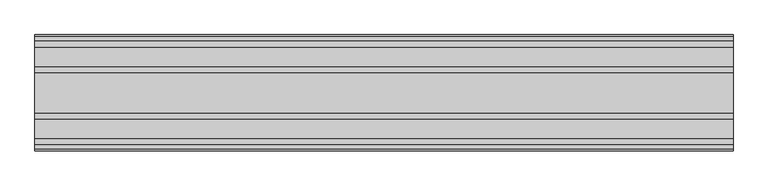
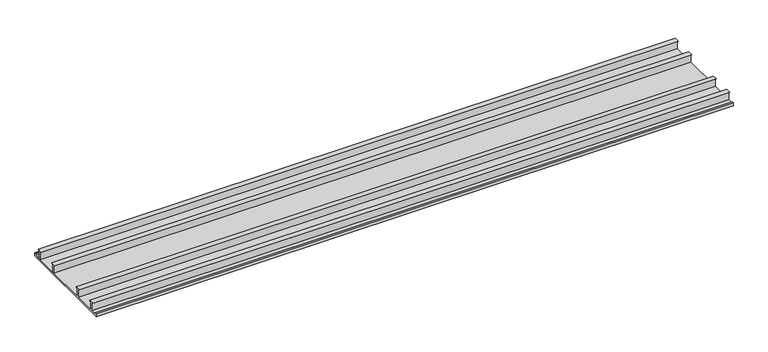
"""IFC4 building model written with IfcOpenShell, lengths in millimetres: proxy geometry, TN_Гидрошпонка ТН Фундамент : Гидрошпонка ТН Фундамент ТШ-Н-250."""

from ifc_helpers import new_model, si_unit, frame, origin, place, context, project, spatial, polyline, outline, extrude, source, transform, mapped, element, save


def specialty_equipment_2380367d(model_context):
    return source(origin(), model_context, "Body", "SweptSolid", [
        extrude(outline(polyline([(125.0, 0.0), (-125.0, 0.0), (-125.0, 7.9804873), (-122.0, 7.9804873), (-122.0, 4.0), (-107.0456593, 4.0), (-107.0456593, 22.012356), (-111.0, 25.0), (-99.0, 25.0), (-102.9543407, 22.012356), (-102.9543407, 4.0), (-52.0456593, 4.0), (-52.0456593, 22.012356), (-56.0, 25.0), (-44.0, 25.0), (-47.9543407, 22.012356), (-47.9543407, 4.0), (47.9543407, 4.0), (47.9543407, 22.012356), (44.0, 25.0), (56.0, 25.0), (52.0456593, 22.012356), (52.0456593, 4.0), (102.9543407, 4.0), (102.9543407, 22.012356), (99.0, 25.0), (111.0, 25.0), (107.0456593, 22.012356), (107.0456593, 4.0), (122.0, 4.0), (122.0, 7.9804873), (125.0, 7.9804873), (125.0, 0.0)])), frame((0.0, 0.0, 0.0), z_axis=(1.0, 0.0, 0.0), x_axis=(0.0, 1.0, 0.0)), (0.0, 0.0, 1.0), 1500.0),
    ])


if __name__ == "__main__":
    model = new_model("IFC4")
    model_context = context("Model", 3, world=origin())
    ifc_project = project(units=[si_unit("LENGTHUNIT", "METRE", prefix="MILLI")], contexts=[model_context])
    site = spatial("IfcSite", under=ifc_project)
    building = spatial("IfcBuilding", under=site)
    placement = place(None, origin())
    specialty_equipment_shape = specialty_equipment_2380367d(model_context)
    element("IfcBuildingElementProxy", 1, Name="TN_Гидрошпонка ТН Фундамент : Гидрошпонка ТН Фундамент ТШ-Н-250", ObjectType="TN_Гидрошпонка ТН Фундамент : Гидрошпонка ТН Фундамент ТШ-Н-250", at=placement, inside=building, context=model_context, shape_type="MappedRepresentation", body=[
        mapped(specialty_equipment_shape, transform((0.0, 0.0, 0.0), x_axis=(1.0, 0.0, 0.0), y_axis=(0.0, 1.0, 0.0), z_axis=(0.0, 0.0, 1.0))),
    ])
    save(model, "model.ifc")

# Revit data of these elements
# Type "TN_Гидрошпонка ТН Фундамент : Гидрошпонка ТН Фундамент ТШ-Н-250"
#   Description = "Наружные гидроизоляционные шпонки ТН Фундамент ТШ-Н предназначены для герметизации технологических швов бетонирования при строительстве подземных и заглубленных конструкций зданий и сооружений различного назначения и класса ответственности."
#   Type Comments = "п.м."
#   Manufacturer = "ТехноНИКОЛЬ"
#   URL = "https://nav.tn.ru/catalog/gidroizolyatsiya/komplektatsiya-dlya-gidroizolyatsii/gidroshponki-tekhnonikol-fundament-tsh-n/"
#   ADSK_Примечание = ""
#   ADSK_Обозначение [instance default] = "ТехноНИКОЛЬ"
#   ADSK_Наименование = "Гидрошпонка ТН Фундамент ТШ-Н-250"
#   ADSK_Масса_Текст = ""
#   ADSK_Марка = ""
#   ADSK_Код изделия = "66673"
#   ADSK_Завод-изготовитель [instance default] = "ТехноНИКОЛЬ"
#   ADSK_Единица измерения [instance default] = "п.м."
#   ADSK_Группирование = "Гидрошпонки"
#   ADSK_URL страницы изделия = "https://nav.tn.ru/catalog/gidroizolyatsiya/komplektatsiya-dlya-gidroizolyatsii/gidroshponki-tekhnonikol-fundament-tsh-n/"
#   ADSK_URL документации изделия = "https://nav.tn.ru/upload/iblock/ff2/kxdk1yskynmm632h8p9i264cjgkfwq9e/Tekhlist-7.402_Gidroshponki-TN-Fundament-TSH_N_RU_ru.pdf"
#   built-in parameter 1001306 [instance default] = 3.28084 (stored number, unit not read)
#   ADSK_Размер_Длина [instance default] = 1000 mm
#   ADSK_Количество [instance default] = 1
#   Гидрошпонка ТН Фундамент ТШ-Н-210 = no
#   Гидрошпонка ТН Фундамент ДШП-В-50 = no
#   Гидрошпонка ТН Фундамент ДШП-В-20 = no
#   Гидрошпонка ТН Фундамент ДШ-В-280 = no
#   Гидрошпонка ТН Фундамент ДШ-В-250 = no
#   Гидрошпонка ТН Фундамент ТШ-В-250 = no
#   Гидрошпонка ТН Фундамент ТПС-В 140-1 = no
#   Гидрошпонка ТН Фундамент ДШ-Н-280 = no
#   Гидрошпонка ТН Фундамент ДШ-Н-250 = no
#   Гидрошпонка ТН Фундамент ТПС-В 100-2 = no
#   Гидрошпонка ТН Фундамент ТШ-Н-250 = yes
#   Гидрошпонка ТН Фундамент ТШ-В-210 = no
#   Материал = TN_ПВХ_Черный
#   Default Elevation = 0
# Element 1 (IfcBuildingElementProxy, "TN_Гидрошпонка ТН Фундамент : Гидрошпонка ТН Фундамент ТШ-Н-250")
#   built-in parameter 1001306 = 4.92126 (stored number, unit not read)
#   ADSK_Размер_Длина = 1500 mm
#   ADSK_Количество = 1.5
#   Materials on its faces: "TN_ПВХ_Черный"
# Materials
#   "TN_ПВХ_Черный": class "Типовые", colour RGB 48 48 48, transparency 0, Cost = 0
